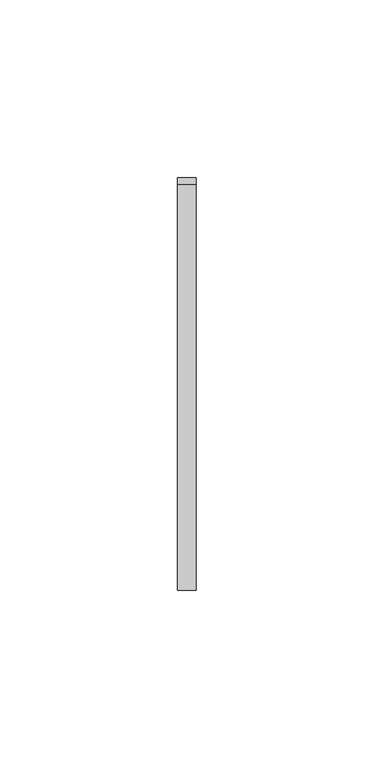
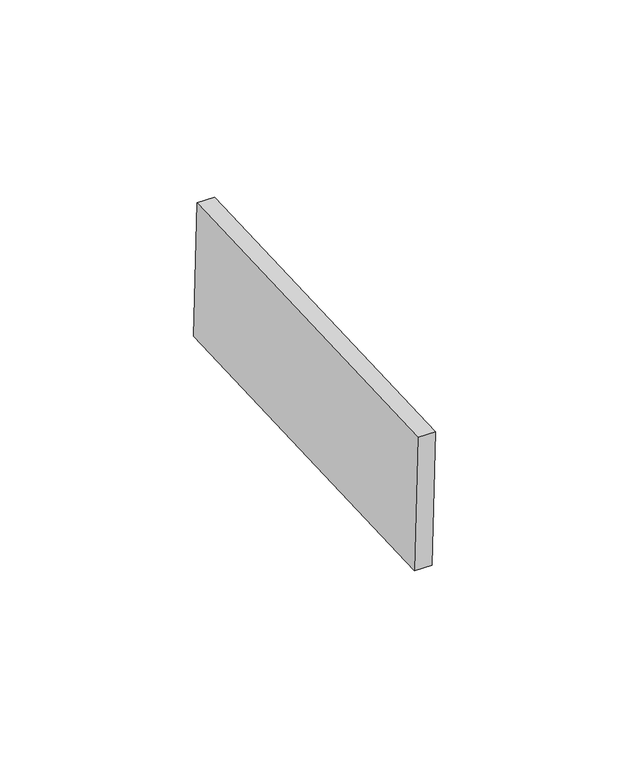
"""IFC4 building model written with IfcOpenShell, lengths in millimetres: proxy geometry, Inner panel:Inner panel:1:Inner panel:1 : Inner panel:Inner panel:300324:2:Inner panel:1:Inner panel:1 : Inner panel:Inner panel:300324:2 : Inner panel:Inner panel:1:Inner panel:1 : Inner panel:Inner panel:300324:300043:96 : Inner panel:Inner panel:1:Inner panel:1 : Inner panel:Inner panel:300324:2:Inner panel:1:Inner panel:1 : Inner panel:Inner panel:300324:2 : Inner panel:Inner panel:1:Inner panel:1 : Inner panel:Inner panel:300324:300043:308120."""

from ifc_helpers import new_model, si_unit, frame, origin, place, context, project, spatial, polyline, outline, extrude, source, transform, mapped, element, save


def generic_models_1184a622(model_context):
    return source(origin(), model_context, "Body", "SweptSolid", [
        extrude(outline(polyline([(0.0, -114.2999999), (0.0, 0.0), (5.2138089, 0.0), (5.2138089, -114.2999999), (0.0, -114.2999999)])), frame((593530.195117, -568168.273882, 8806.9397902), z_axis=(0.0, -0.04163054471215927, 0.9991330730923529), x_axis=(-1.0, 0.0, 0.0)), (0.0, 0.0, 1.0), 43.2233908),
    ])


if __name__ == "__main__":
    model = new_model("IFC4")
    model_context = context("Model", 3, world=origin())
    ifc_project = project(units=[si_unit("LENGTHUNIT", "METRE", prefix="MILLI")], contexts=[model_context])
    site = spatial("IfcSite", under=ifc_project)
    building = spatial("IfcBuilding", under=site)
    placement = place(None, origin())
    generic_models_shape = generic_models_1184a622(model_context)
    element("IfcBuildingElementProxy", 1, Name="Inner panel:Inner panel:1:Inner panel:1 : Inner panel:Inner panel:300324:2:Inner panel:1:Inner panel:1 : Inner panel:Inner panel:300324:2 : Inner panel:Inner panel:1:Inner panel:1 : Inner panel:Inner panel:300324:300043:96 : Inner panel:Inner panel:1:Inner panel:1 : Inner panel:Inner panel:300324:2:Inner panel:1:Inner panel:1 : Inner panel:Inner panel:300324:2 : Inner panel:Inner panel:1:Inner panel:1 : Inner panel:Inner panel:300324:300043:308120", ObjectType="Inner panel:Inner panel:1:Inner panel:1 : Inner panel:Inner panel:300324:2:Inner panel:1:Inner panel:1 : Inner panel:Inner panel:300324:2 : Inner panel:Inner panel:1:Inner panel:1 : Inner panel:Inner panel:300324:300043:96 : Inner panel:Inner panel:1:Inner panel:1 : Inner panel:Inner panel:300324:2:Inner panel:1:Inner panel:1 : Inner panel:Inner panel:300324:2 : Inner panel:Inner panel:1:Inner panel:1 : Inner panel:Inner panel:300324:300043:308120", at=placement, inside=building, context=model_context, shape_type="MappedRepresentation", body=[
        mapped(generic_models_shape, transform((0.0, 0.0, 0.0), x_axis=(1.0, 0.0, 0.0), y_axis=(0.0, 1.0, 0.0), z_axis=(0.0, 0.0, 1.0))),
    ])
    save(model, "model.ifc")

# Revit data of these elements
# Type "Inner panel:Inner panel:1:Inner panel:1 : Inner panel:Inner panel:300324:2:Inner panel:1:Inner panel:1 : Inner panel:Inner panel:300324:2 : Inner panel:Inner panel:1:Inner panel:1 : Inner panel:Inner panel:300324:300043:96 : Inner panel:Inner panel:1:Inner panel:1 : Inner panel:Inner panel:300324:2:Inner panel:1:Inner panel:1 : Inner panel:Inner panel:300324:2 : Inner panel:Inner panel:1:Inner panel:1 : Inner panel:Inner panel:300324:300043:308120"
#   NameOverride = "Inner panel:Inner panel:1:Inner panel:1 : Inner panel:Inner panel:300324:2:Inner panel:1:Inner panel:1 : Inner panel:Inner panel:300324:2 : Inner panel:Inner panel:1:Inner panel:1 : Inner panel:Inner panel:300324:300043:308120"
#   ObjectTypeOverride = "Inner panel:1:Inner panel:1 : Inner panel:Inner panel:300324:2 : Inner panel:Inner panel:1:Inner panel:1 : Inner panel:Inner panel:300324:300043"
#   Reference = "Inner panel"
#   Tag = "308120"
# Element 1 (IfcBuildingElementProxy, "Inner panel:Inner panel:1:Inner panel:1 : Inner panel:Inner panel:300324:2:Inner panel:1:Inner panel:1 : Inner panel:Inner panel:300324:2 : Inner panel:Inner panel:1:Inner panel:1 : Inner panel:Inner panel:300324:300043:96 : Inner panel:Inner panel:1:Inner panel:1 : Inner panel:Inner panel:300324:2:Inner panel:1:Inner panel:1 : Inner panel:Inner panel:300324:2 : Inner panel:Inner panel:1:Inner panel:1 : Inner panel:Inner panel:300324:300043:308120")
#   Materials on its faces: "SLIDING CLIP"
# Materials
#   "SLIDING CLIP": class "Generic", colour RGB 120 120 120, transparency 0, Cost = 0
